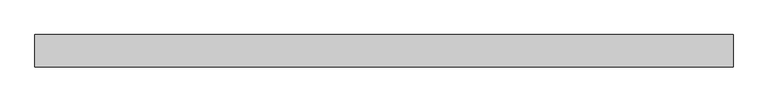
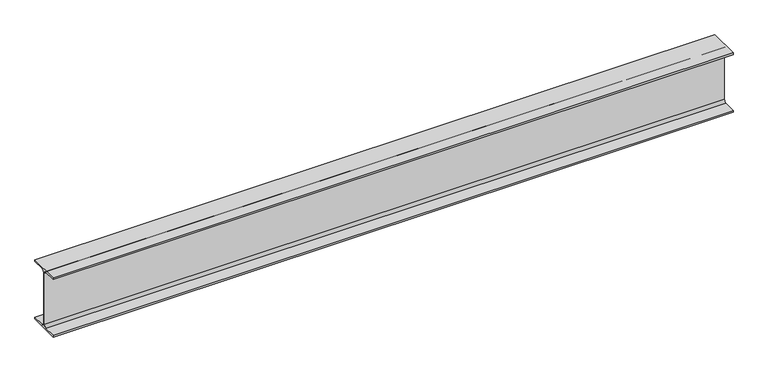
"""IFC4 building model written with IfcOpenShell, lengths in millimetres: beam geometry, Steel Framing_H_KS : H_SB_AR_S02_H-300x150x6.5x9_WG1."""

from ifc_helpers import new_model, si_unit, point, frame, frame_2d, origin, place, context, project, spatial, polyline, circle_curve, trimmed, segment, composite_curve, outline, extrude, source, transform, mapped, element, save


def beam_6c4fcb1b(model_context):
    return source(origin(), model_context, "Body", "SweptSolid", [
        extrude(outline(composite_curve([segment(polyline([(75.0, -141.0), (75.0, -150.0), (-75.0, -150.0), (-75.0, -141.0), (-16.25, -141.0)]), True, "CONTINUOUS"), segment(trimmed(circle_curve(frame_2d((-16.25, -128.0)), 13.0), [point((-16.25, -141.0))], [point((-3.25, -128.0))], True, "CARTESIAN"), True, "CONTINUOUS"), segment(polyline([(-3.25, -128.0), (-3.25, 128.0)]), True, "CONTINUOUS"), segment(trimmed(circle_curve(frame_2d((-16.25, 128.0)), 13.0), [point((-3.25, 128.0))], [point((-16.25, 141.0))], True, "CARTESIAN"), True, "CONTINUOUS"), segment(polyline([(-16.25, 141.0), (-75.0, 141.0), (-75.0, 150.0), (75.0, 150.0), (75.0, 141.0), (16.25, 141.0)]), True, "CONTINUOUS"), segment(trimmed(circle_curve(frame_2d((16.25, 128.0)), 13.0), [point((16.25, 141.0))], [point((3.25, 128.0))], True, "CARTESIAN"), True, "CONTINUOUS"), segment(polyline([(3.25, 128.0), (3.25, -128.0)]), True, "CONTINUOUS"), segment(trimmed(circle_curve(frame_2d((16.25, -128.0)), 13.0), [point((3.25, -128.0))], [point((16.25, -141.0))], True, "CARTESIAN"), True, "CONTINUOUS"), segment(polyline([(16.25, -141.0), (75.0, -141.0)]), True, "CONTINUOUS")], self_intersect=False)), frame((-1662.3, 0.0, 0.0), z_axis=(1.0, 0.0, 0.0), x_axis=(0.0, 1.0, 0.0)), (0.0, 0.0, 1.0), 3249.6),
    ])


if __name__ == "__main__":
    model = new_model("IFC4")
    model_context = context("Model", 3, world=origin())
    ifc_project = project(units=[si_unit("LENGTHUNIT", "METRE", prefix="MILLI")], contexts=[model_context])
    site = spatial("IfcSite", under=ifc_project)
    building = spatial("IfcBuilding", under=site)
    placement = place(None, origin())
    beam_shape = beam_6c4fcb1b(model_context)
    element("IfcBeam", 1, ObjectType="Steel Framing_H_KS : H_SB_AR_S02_H-300x150x6.5x9_WG1", at=placement, inside=building, context=model_context, shape_type="MappedRepresentation", body=[
        mapped(beam_shape, transform((0.0, 0.0, 0.0), x_axis=(1.0, 0.0, 0.0), y_axis=(0.0, 1.0, 0.0), z_axis=(0.0, 0.0, 1.0))),
    ])
    save(model, "model.ifc")

# Revit data of these elements
# Type "Steel Framing_H_KS : H_SB_AR_S02_H-300x150x6.5x9_WG1"
#   Type Comments = "MAIN"
#   Type Mark = "WG1"
#   H_SectionID = "H-300x150x6.5x9"
#   H_Ratio for Additional Steel Plate = 0.2
#   Width = 15.0 cm
#   Web Thickness = 0.65 cm
#   Web Fillet = 1.3 cm
#   Warping Constant = 107000.0 cm⁶
#   Torsional Moment of Inertia = 9.9539 cm⁴
#   Section Area = 46.78 cm²
#   Plastic Modulus weak axis = 105.0 cm³
#   Plastic Modulus strong axis = 542.0 cm³
#   Perimeter = 1.17 m²/m
#   Nominal Weight = 36.70 kgf/m
#   Moment of Inertia weak axis = 508.00 cm⁴
#   Moment of Inertia strong axis = 7210.00 cm⁴
#   Height = 30.0 cm
#   Flange Thickness = 0.9 cm
#   Elastic Modulus weak axis = 67.7 cm³
#   Elastic Modulus strong axis = 481.0 cm³
#   Centroid Vertical = 15.0 cm
#   Centroid Horizontal = 7.5 cm
#   Bolt Spacing = 8.89 cm
#   Length [instance default] = 1500 mm
#   Structural Material [instance default] = Steel, 45-345
#   Section Name Key = ""
#   Assembly Code = ""
# Element 1 (IfcBeam, "Steel Framing_H_KS : H_SB_AR_S02_H-300x150x6.5x9_WG1")
#   Materials on its faces: "Steel, 45-345"
# Materials
#   "Steel, 45-345": class "Metal", colour RGB 189 187 185, transparency 0, Description = "Steel 345 MPa", Cost = 0
